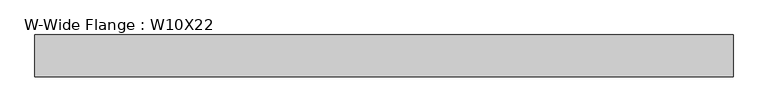
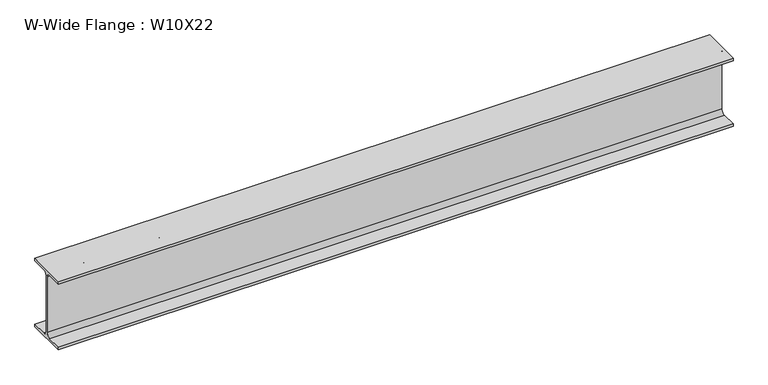
"""IFC4 building model written with IfcOpenShell, lengths in millimetres: beam geometry, W-Wide Flange : W10X22."""

from ifc_helpers import new_model, si_unit, point, frame, frame_2d, origin, place, context, project, spatial, polyline, circle_curve, trimmed, segment, composite_curve, outline, extrude, source, transform, mapped, element, save


def w_wide_flange_w10x22_9a287cc3(model_context):
    return source(origin(), model_context, "Body", "SweptSolid", [
        extrude(outline(composite_curve([segment(polyline([(73.025, -120.396), (73.025, -129.54), (-73.025, -129.54), (-73.025, -120.396), (-17.7165, -120.396)]), True, "CONTINUOUS"), segment(trimmed(circle_curve(frame_2d((-17.7165, -105.7275)), 14.6685), [point((-17.7165, -120.396))], [point((-3.048, -105.7275))], True, "CARTESIAN"), True, "CONTINUOUS"), segment(polyline([(-3.048, -105.7275), (-3.048, 105.7275)]), True, "CONTINUOUS"), segment(trimmed(circle_curve(frame_2d((-17.7165, 105.7275)), 14.6685), [point((-3.048, 105.7275))], [point((-17.7165, 120.396))], True, "CARTESIAN"), True, "CONTINUOUS"), segment(polyline([(-17.7165, 120.396), (-73.025, 120.396), (-73.025, 129.54), (73.025, 129.54), (73.025, 120.396), (17.7165, 120.396)]), True, "CONTINUOUS"), segment(trimmed(circle_curve(frame_2d((17.7165, 105.7275)), 14.6685), [point((17.7165, 120.396))], [point((3.048, 105.7275))], True, "CARTESIAN"), True, "CONTINUOUS"), segment(polyline([(3.048, 105.7275), (3.048, -105.7275)]), True, "CONTINUOUS"), segment(trimmed(circle_curve(frame_2d((17.7165, -105.7275)), 14.6685), [point((3.048, -105.7275))], [point((17.7165, -120.396))], True, "CARTESIAN"), True, "CONTINUOUS"), segment(polyline([(17.7165, -120.396), (73.025, -120.396)]), True, "CONTINUOUS")], self_intersect=False)), frame((-1170.1145, 0.0, 0.0), z_axis=(1.0, 0.0, 0.0), x_axis=(0.0, 1.0, 0.0)), (0.0, 0.0, 1.0), 2425.954),
    ])


if __name__ == "__main__":
    model = new_model("IFC4")
    model_context = context("Model", 3, world=origin())
    ifc_project = project(units=[si_unit("LENGTHUNIT", "METRE", prefix="MILLI")], contexts=[model_context])
    site = spatial("IfcSite", under=ifc_project)
    building = spatial("IfcBuilding", under=site)
    placement = place(None, origin())
    w_wide_flange_w10x22_shape = w_wide_flange_w10x22_9a287cc3(model_context)
    element("IfcBeam", 1, ObjectType="W-Wide Flange : W10X22", at=placement, inside=building, context=model_context, shape_type="MappedRepresentation", body=[
        mapped(w_wide_flange_w10x22_shape, transform((0.0, 0.0, 0.0), x_axis=(1.0, 0.0, 0.0), y_axis=(0.0, 1.0, 0.0), z_axis=(0.0, 0.0, 1.0))),
    ])
    save(model, "model.ifc")

# Revit data of these elements
# Type "W-Wide Flange : W10X22"
#   Assembly Code = "B10"
#   W = 22
#   Length [instance default] = 5' - 0"
#   bf = 0' - 5 3/4"
#   d = 0' - 10.2"
#   k = 0' - 0 15/16"
#   k2 = 0' - 0.5775"
#   tf = 0' - 0.36"
#   tw = 0' - 0.24"
#   A = 0.0450694 SF
#   Structural Material [instance default] = _STRUCTURAL STEEL (SEE STRUCT. DWGS)
# Element 1 (IfcBeam, "W-Wide Flange : W10X22")
#   Materials on its faces: "_STRUCTURAL STEEL (SEE STRUCT. DWGS)"
# Materials
#   "_STRUCTURAL STEEL (SEE STRUCT. DWGS)": class "Metal", colour RGB 199 199 199, transparency 0, Description = "Structural steel 50ksi", Cost = 0
